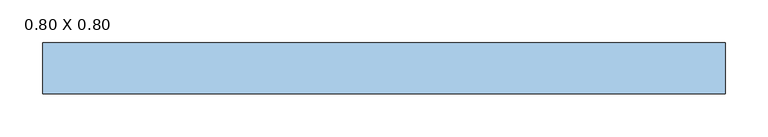
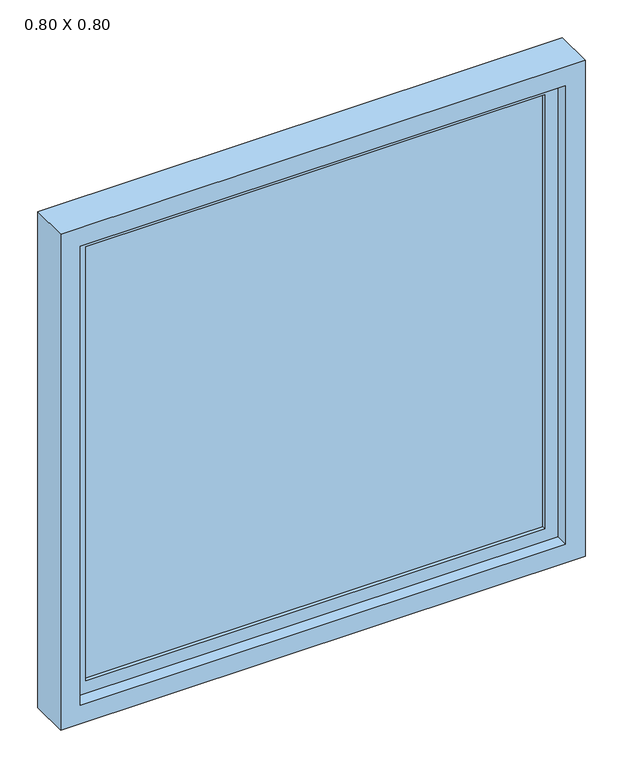
"""IFC4 building model written with IfcOpenShell, lengths in millimetres: window geometry, .CC_ND 300_MAXIM-AR : 0.80 X 0.80."""

from ifc_helpers import new_model, si_unit, frame, origin, place, context, project, spatial, polyline, outline, extrude, source, transform, mapped, element, save


def window_0_80_x_0_80_067849bc(model_context):
    return source(origin(), model_context, "Body", "SweptSolid", [
        extrude(outline(polyline([(-350.0, -4.0), (-350.0, 4.0), (350.0, 4.0), (350.0, -4.0), (-350.0, -4.0)])), frame((0.0, 0.0, 1550.0), z_axis=(0.0, 0.0, 1.0), x_axis=(1.0, 0.0, 0.0)), (0.0, 0.0, 1.0), 700.0),
        extrude(outline(polyline([(1530.0, 370.0), (2270.0, 370.0), (2270.0, -370.0), (1530.0, -370.0), (1530.0, 370.0)]), holes=[polyline([(2250.0, 350.0), (1550.0, 350.0), (1550.0, -350.0), (2250.0, -350.0), (2250.0, 350.0)])]), frame((0.0, -10.0, 0.0), z_axis=(0.0, 1.0, 0.0), x_axis=(0.0, 0.0, 1.0)), (0.0, 0.0, 1.0), 20.0),
        extrude(outline(polyline([(1500.0, 400.0), (2300.0, 400.0), (2300.0, -400.0), (1500.0, -400.0), (1500.0, 400.0)]), holes=[polyline([(2270.0, 370.0), (1530.0, 370.0), (1530.0, -370.0), (2270.0, -370.0), (2270.0, 370.0)])]), frame((0.0, -30.0, 0.0), z_axis=(0.0, 1.0, 0.0), x_axis=(0.0, 0.0, 1.0)), (0.0, 0.0, 1.0), 60.0),
    ])


if __name__ == "__main__":
    model = new_model("IFC4")
    model_context = context("Model", 3, world=origin())
    ifc_project = project(units=[si_unit("LENGTHUNIT", "METRE", prefix="MILLI")], contexts=[model_context])
    site = spatial("IfcSite", under=ifc_project)
    building = spatial("IfcBuilding", under=site)
    placement = place(None, origin())
    window_0_80_x_0_80_shape = window_0_80_x_0_80_067849bc(model_context)
    element("IfcWindow", 1, ObjectType=".CC_ND 300_MAXIM-AR : 0.80 X 0.80", at=placement, inside=building, context=model_context, shape_type="MappedRepresentation", body=[
        mapped(window_0_80_x_0_80_shape, transform((0.0, 0.0, 0.0), x_axis=(1.0, 0.0, 0.0), y_axis=(0.0, 1.0, 0.0), z_axis=(0.0, 0.0, 1.0))),
    ])
    save(model, "model.ifc")

# Revit data of these elements
# Type ".CC_ND 300_MAXIM-AR : 0.80 X 0.80"
#   Type Mark = "65"
#   Largura Painel [instance default] = 0.02 m
#   Largura Esquadria [instance default] = 0.06 m
#   Espessura Vidro [instance default] = 0.008 m
#   Espessura Painel [instance default] = 0.02 m
#   Espessura Esquadria [instance default] = 0.03 m
#   Height = 0.80 m
#   Altura-padrão do peitoril = 1.50 m
#   Width = 0.80 m
#   Vidro = .VIDRO GENÉRICO
#   Esquadria = .ALUMÍNIO COM PINTURA ELETROSTÁTICA BRANCA
#   Wall Closure = (empty or 0)
# Element 1 (IfcWindow, ".CC_ND 300_MAXIM-AR : 0.80 X 0.80")
#   Materials on its faces: ".ALUMÍNIO COM PINTURA ELETROSTÁTICA BRANCA", ".VIDRO GENÉRICO"
# Materials
#   ".VIDRO GENÉRICO": class ".CC_VIDRO", colour RGB 0 128 192, transparency 0.9, Description = "Vidro comum", Cost = 0
#   ".ALUMÍNIO COM PINTURA ELETROSTÁTICA BRANCA": class "CC_METAIS", colour RGB 241 241 241, transparency 0, Cost = 0
